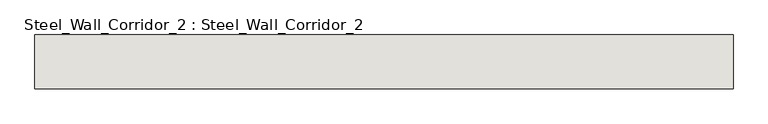
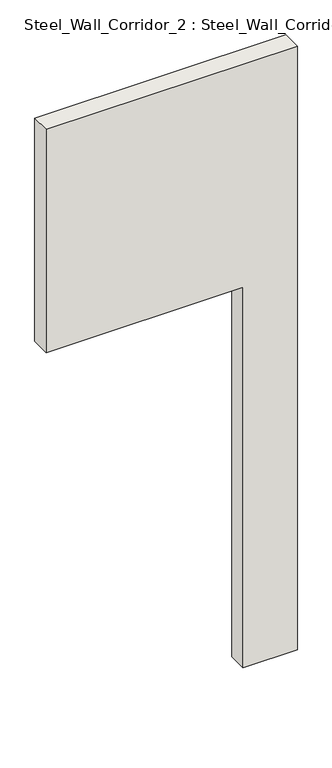
"""IFC4 building model written with IfcOpenShell, lengths in millimetres: wall geometry, Steel_Wall_Corridor_2 : Steel_Wall_Corridor_2."""

from ifc_helpers import new_model, si_unit, frame, origin, place, context, project, spatial, polyline, outline, extrude, source, transform, mapped, element, save


def steel_wall_corridor_2_steel_wall_corridor_2_3c3fb1a4(model_context):
    return source(origin(), model_context, "Body", "SweptSolid", [
        extrude(outline(polyline([(3550.0, 1515.0), (3550.0, 215.0), (2330.0, 215.0), (2330.0, 1235.0), (250.0, 1235.0), (250.0, 1515.0), (3550.0, 1515.0)])), frame((0.0, 9495.0, 0.0), z_axis=(0.0, 1.0, 0.0), x_axis=(0.0, 0.0, 1.0)), (0.0, 0.0, 1.0), 100.0),
    ])


if __name__ == "__main__":
    model = new_model("IFC4")
    model_context = context("Model", 3, world=origin())
    ifc_project = project(units=[si_unit("LENGTHUNIT", "METRE", prefix="MILLI")], contexts=[model_context])
    site = spatial("IfcSite", under=ifc_project)
    building = spatial("IfcBuilding", under=site)
    placement = place(None, origin())
    steel_wall_corridor_2_steel_wall_corridor_2_shape = steel_wall_corridor_2_steel_wall_corridor_2_3c3fb1a4(model_context)
    element("IfcWall", 1, ObjectType="Steel_Wall_Corridor_2 : Steel_Wall_Corridor_2", at=placement, inside=building, context=model_context, shape_type="MappedRepresentation", body=[
        mapped(steel_wall_corridor_2_steel_wall_corridor_2_shape, transform((0.0, 0.0, 0.0), x_axis=(1.0, 0.0, 0.0), y_axis=(0.0, 1.0, 0.0), z_axis=(0.0, 0.0, 1.0))),
    ])
    save(model, "model.ifc")

# Revit data of these elements
# Type "Steel_Wall_Corridor_2 : Steel_Wall_Corridor_2"
#   NameOverride = "Steel_Wall_Corridor_2"
# Element 1 (IfcWall, "Steel_Wall_Corridor_2 : Steel_Wall_Corridor_2")
#   Materials on its faces: "IfcSurfaceStyle #33"
# Materials
#   "IfcSurfaceStyle #33": class "Unassigned", colour RGB 214 214 214, transparency 0
